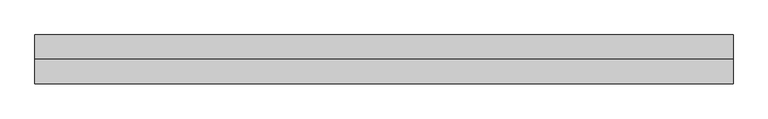
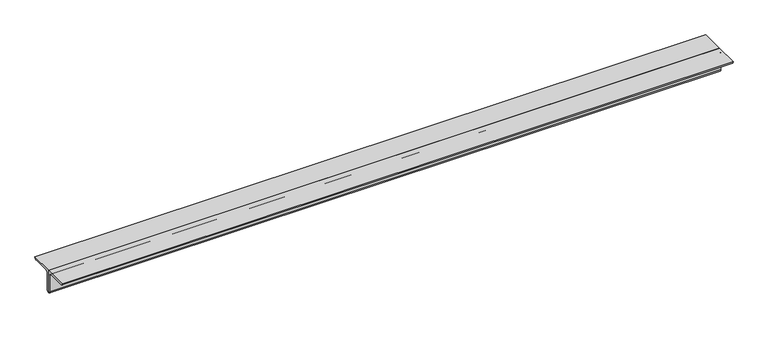
"""IFC4 building model written with IfcOpenShell, lengths in millimetres: member geometry, 0123_Steel Framing_2Ls-KSD3502 : H_SB_AR_S03_2Ls-130x130x12_HBR1."""

from ifc_helpers import new_model, si_unit, point, frame, frame_2d, origin, place, context, project, spatial, polyline, circle_curve, trimmed, segment, composite_curve, outline, extrude, source, transform, mapped, element, save


def member_70dd3ef8(model_context):
    return source(origin(), model_context, "Body", "SweptSolid", [
        extrude(outline(composite_curve([segment(polyline([(0.0, 36.4), (0.0, -93.6)]), True, "CONTINUOUS"), segment(trimmed(circle_curve(frame_2d((0.0, -81.6)), 12.0), [point((0.0, -93.6))], [point((-12.0, -81.6))], False, "CARTESIAN"), True, "CONTINUOUS"), segment(polyline([(-12.0, -81.6), (-12.0, 12.4)]), True, "CONTINUOUS"), segment(trimmed(circle_curve(frame_2d((-24.0, 12.4)), 12.0), [point((-12.0, 12.4))], [point((-24.0, 24.4))], True, "CARTESIAN"), True, "CONTINUOUS"), segment(polyline([(-24.0, 24.4), (-118.0, 24.4)]), True, "CONTINUOUS"), segment(trimmed(circle_curve(frame_2d((-118.0, 36.4)), 12.0), [point((-118.0, 24.4))], [point((-130.0, 36.4))], False, "CARTESIAN"), True, "CONTINUOUS"), segment(polyline([(-130.0, 36.4), (0.0, 36.4)]), True, "CONTINUOUS")], self_intersect=False)), frame((-1844.6975967, 0.0, 0.0), z_axis=(1.0, 0.0, 0.0), x_axis=(0.0, 1.0, 0.0)), (0.0, 0.0, 1.0), 3701.6272171),
        extrude(outline(composite_curve([segment(polyline([(0.0, 36.4), (130.0, 36.4)]), True, "CONTINUOUS"), segment(trimmed(circle_curve(frame_2d((118.0, 36.4)), 12.0), [point((130.0, 36.4))], [point((118.0, 24.4))], False, "CARTESIAN"), True, "CONTINUOUS"), segment(polyline([(118.0, 24.4), (24.0, 24.4)]), True, "CONTINUOUS"), segment(trimmed(circle_curve(frame_2d((24.0, 12.4)), 12.0), [point((24.0, 24.4))], [point((12.0, 12.4))], True, "CARTESIAN"), True, "CONTINUOUS"), segment(polyline([(12.0, 12.4), (12.0, -81.6)]), True, "CONTINUOUS"), segment(trimmed(circle_curve(frame_2d((0.0, -81.6)), 12.0), [point((12.0, -81.6))], [point((0.0, -93.6))], False, "CARTESIAN"), True, "CONTINUOUS"), segment(polyline([(0.0, -93.6), (0.0, 36.4)]), True, "CONTINUOUS")], self_intersect=False)), frame((-1844.6975967, 0.0, 0.0), z_axis=(1.0, 0.0, 0.0), x_axis=(0.0, 1.0, 0.0)), (0.0, 0.0, 1.0), 3701.6272171),
    ])


if __name__ == "__main__":
    model = new_model("IFC4")
    model_context = context("Model", 3, world=origin())
    ifc_project = project(units=[si_unit("LENGTHUNIT", "METRE", prefix="MILLI")], contexts=[model_context])
    site = spatial("IfcSite", under=ifc_project)
    building = spatial("IfcBuilding", under=site)
    placement = place(None, origin())
    member_shape = member_70dd3ef8(model_context)
    element("IfcMember", 1, ObjectType="0123_Steel Framing_2Ls-KSD3502 : H_SB_AR_S03_2Ls-130x130x12_HBR1", at=placement, inside=building, context=model_context, shape_type="MappedRepresentation", body=[
        mapped(member_shape, transform((0.0, 0.0, 0.0), x_axis=(1.0, 0.0, 0.0), y_axis=(0.0, 1.0, 0.0), z_axis=(0.0, 0.0, 1.0))),
    ])
    save(model, "model.ifc")

# Revit data of these elements
# Type "0123_Steel Framing_2Ls-KSD3502 : H_SB_AR_S03_2Ls-130x130x12_HBR1"
#   Type Mark = "HBR1"
#   Assembly Code = "B10"
#   Legs = "SLBB"
#   W = 8.97
#   Perimeter = 1.04 m²/m
#   Nominal Weight = 46.80 kgf/m
#   Length [instance default] = 1000 mm
#   Space = 0 mm
#   b = 130 mm
#   d = 130 mm
#   t = 12 mm
#   y = 36.4 mm
#   A = 0.005952 m²
#   Structural Material [instance default] = Steel ASTM A36
# Element 1 (IfcMember, "0123_Steel Framing_2Ls-KSD3502 : H_SB_AR_S03_2Ls-130x130x12_HBR1")
#   Materials on its faces: "Steel ASTM A36"
# Materials
#   "Steel ASTM A36": class "Metal", colour RGB 199 199 199, transparency 0, Description = "Structural steel, ASTM A36 Grade B, mill finish", Cost = 0
